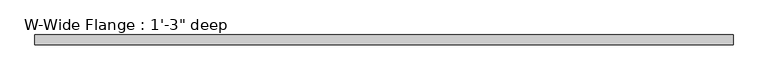
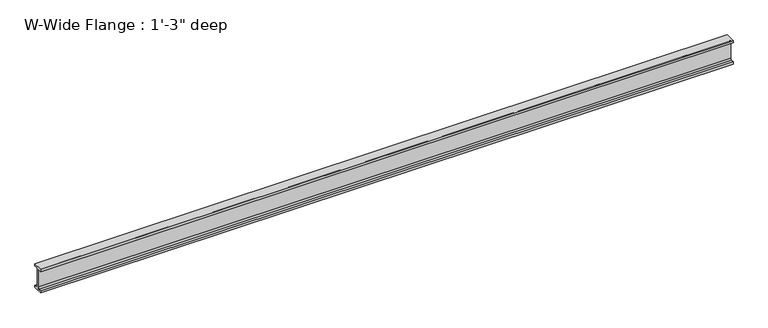
"""IFC4 building model written with IfcOpenShell, lengths in millimetres: beam geometry."""

from ifc_helpers import new_model, si_unit, point, frame, frame_2d, origin, place, context, project, spatial, polyline, circle_curve, trimmed, segment, composite_curve, outline, extrude, source, transform, mapped, element, save


def beam_c3201f3b(model_context):
    return source(origin(), model_context, "Body", "SweptSolid", [
        extrude(outline(composite_curve([segment(polyline([(76.2, -155.956), (76.2, -190.5), (-76.2, -190.5), (-76.2, -155.956), (-32.131, -155.956)]), True, "CONTINUOUS"), segment(trimmed(circle_curve(frame_2d((-32.131, -133.35)), 22.606), [point((-32.131, -155.956))], [point((-9.525, -133.35))], True, "CARTESIAN"), True, "CONTINUOUS"), segment(polyline([(-9.525, -133.35), (-9.525, 133.35)]), True, "CONTINUOUS"), segment(trimmed(circle_curve(frame_2d((-32.131, 133.35)), 22.606), [point((-9.525, 133.35))], [point((-32.131, 155.956))], True, "CARTESIAN"), True, "CONTINUOUS"), segment(polyline([(-32.131, 155.956), (-76.2, 155.956), (-76.2, 190.5), (76.2, 190.5), (76.2, 155.956), (32.131, 155.956)]), True, "CONTINUOUS"), segment(trimmed(circle_curve(frame_2d((32.131, 133.35)), 22.606), [point((32.131, 155.956))], [point((9.525, 133.35))], True, "CARTESIAN"), True, "CONTINUOUS"), segment(polyline([(9.525, 133.35), (9.525, -133.35)]), True, "CONTINUOUS"), segment(trimmed(circle_curve(frame_2d((32.131, -133.35)), 22.606), [point((9.525, -133.35))], [point((32.131, -155.956))], True, "CARTESIAN"), True, "CONTINUOUS"), segment(polyline([(32.131, -155.956), (76.2, -155.956)]), True, "CONTINUOUS")], self_intersect=False)), frame((-5246.0574649, 0.0, 0.0), z_axis=(1.0, 0.0, 0.0), x_axis=(0.0, 1.0, 0.0)), (0.0, 0.0, 1.0), 10639.8071837),
    ])


if __name__ == "__main__":
    model = new_model("IFC4")
    model_context = context("Model", 3, world=origin())
    ifc_project = project(units=[si_unit("LENGTHUNIT", "METRE", prefix="MILLI")], contexts=[model_context])
    site = spatial("IfcSite", under=ifc_project)
    building = spatial("IfcBuilding", under=site)
    placement = place(None, origin())
    beam_shape = beam_c3201f3b(model_context)
    element("IfcBeam", 1, ObjectType="W-Wide Flange : 1'-3\" deep", at=placement, inside=building, context=model_context, shape_type="MappedRepresentation", body=[
        mapped(beam_shape, transform((0.0, 0.0, 0.0), x_axis=(1.0, 0.0, 0.0), y_axis=(0.0, 1.0, 0.0), z_axis=(0.0, 0.0, 1.0))),
    ])
    save(model, "model.ifc")

# Revit data of these elements
# Type "W-Wide Flange : 1'-3\" deep"
#   Assembly Code = "B10"
#   W = 166
#   Length [instance default] = 5' - 0"
#   bf = 0' - 6"
#   d = 1' - 3"
#   k = 0' - 2 1/4"
#   k2 = 0' - 0.89"
#   tf = 0' - 1.36"
#   tw = 0' - 0 3/4"
#   A = 0.338889 SF
#   Structural Material [instance default] = Steel ASTM A992
# Element 1 (IfcBeam, "W-Wide Flange : 1'-3\" deep")
#   Structural Material = STRUCTURAL STEEL - SEE STRUCT. DWGS
#   Materials on its faces: "STRUCTURAL STEEL - SEE STRUCT. DWGS"
# Materials
#   "Steel ASTM A992": class "Metal", colour RGB 199 199 199, transparency 0, Description = "Structural steel 50ksi", Cost = 0
#   "STRUCTURAL STEEL - SEE STRUCT. DWGS": class "Metal", colour RGB 137 146 153, transparency 0, Description = "Steel, mill finish", Cost = 0
